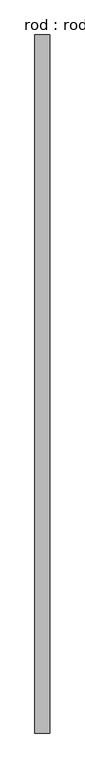
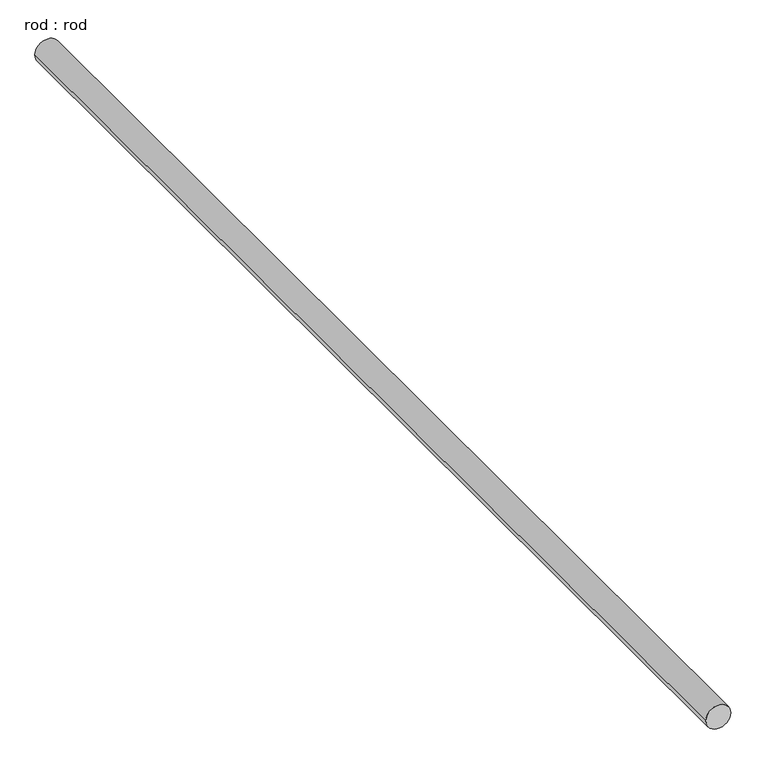
"""IFC4 building model written with IfcOpenShell, lengths in millimetres: proxy geometry, rod : rod."""

from ifc_helpers import new_model, si_unit, point, frame, frame_2d, origin, place, context, project, spatial, circle_curve, trimmed, segment, composite_curve, outline, extrude, source, transform, mapped, element, save


def rod_rod_c1ab920a(model_context):
    return source(origin(), model_context, "Body", "SweptSolid", [
        extrude(outline(composite_curve([segment(trimmed(circle_curve(frame_2d((0.0108462, 0.0)), 200.0), [point((0.0108462, 200.0))], [point((0.0108462, -200.0))], False, "CARTESIAN"), True, "CONTINUOUS"), segment(trimmed(circle_curve(frame_2d((0.0108462, 0.0)), 200.0), [point((0.0108462, -200.0))], [point((0.0108462, 200.0))], False, "CARTESIAN"), True, "CONTINUOUS")], self_intersect=False)), frame((0.0, -5282.2713847, 0.0), z_axis=(0.0, 1.0, 0.0), x_axis=(0.0, 0.0, 1.0)), (0.0, 0.0, 1.0), 18750.0),
    ])


if __name__ == "__main__":
    model = new_model("IFC4")
    model_context = context("Model", 3, world=origin())
    ifc_project = project(units=[si_unit("LENGTHUNIT", "METRE", prefix="MILLI")], contexts=[model_context])
    site = spatial("IfcSite", under=ifc_project)
    building = spatial("IfcBuilding", under=site)
    placement = place(None, origin())
    rod_rod_shape = rod_rod_c1ab920a(model_context)
    element("IfcBuildingElementProxy", 1, Name="rod : rod", ObjectType="rod : rod", at=placement, inside=building, context=model_context, shape_type="MappedRepresentation", body=[
        mapped(rod_rod_shape, transform((0.0, 0.0, 0.0), x_axis=(1.0, 0.0, 0.0), y_axis=(0.0, 1.0, 0.0), z_axis=(0.0, 0.0, 1.0))),
    ])
    save(model, "model.ifc")

# Revit data of these elements
# Type "rod : rod"
#   Default Elevation = 0
